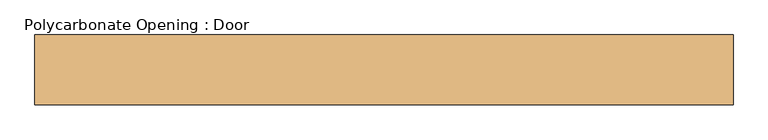
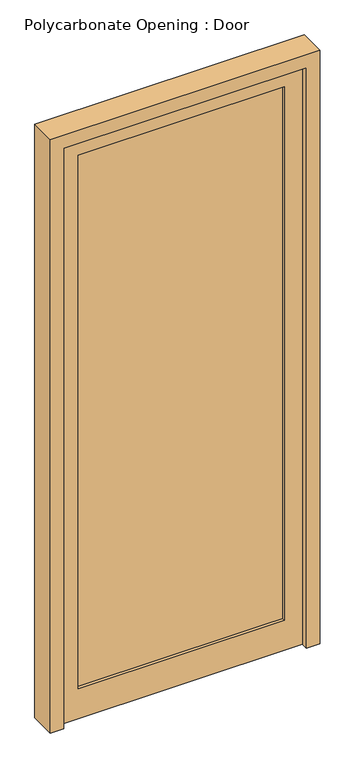
"""IFC4 building model written with IfcOpenShell, lengths in millimetres: door geometry, Polycarbonate Opening : Door."""

import ifcopenshell
import ifcopenshell.guid

model = None  # the IFC model being written
_history = None  # IfcOwnerHistory: only IFC2X3 demands one
_inside = {}  # id of a spatial element -> (the spatial element, [elements in it])
_under = {}  # id of a project, library or spatial element -> (it, [spatial elements below it])
_declared = {}  # id of a project -> (the project, [libraries it declares])
_typed = {}  # id of a type object -> (the type object, [elements of that type])
_made_of = {}  # id of a material, layer set ... -> (it, [elements and type objects made of it])


def new_model(schema):
    """Start an empty IFC model of exactly this schema.

    Asked for "IFC4X3", IfcOpenShell would pick the latest addendum, in which some entities
    have other attributes; the version numbers below select the first issue.
    IFC2X3 requires an IfcOwnerHistory on every rooted entity: one is made here for all.
    """
    global model, _history
    if schema == "IFC4X3":
        model = ifcopenshell.file(schema_version=(4, 3, 0, 0))
    else:
        model = ifcopenshell.file(schema=schema)
    _inside.clear()
    _under.clear()
    _declared.clear()
    _typed.clear()
    _made_of.clear()
    _history = None
    if model.schema == "IFC2X3":
        org = make("IfcOrganization", Name="unknown")
        user = make(
            "IfcPersonAndOrganization",
            ThePerson=make("IfcPerson", FamilyName="unknown"),
            TheOrganization=org,
        )
        app = make(
            "IfcApplication",
            ApplicationDeveloper=org,
            Version="unknown",
            ApplicationFullName="unknown",
            ApplicationIdentifier="unknown",
        )
        _history = make(
            "IfcOwnerHistory",
            OwningUser=user,
            OwningApplication=app,
            ChangeAction="ADDED",
            CreationDate=0,
        )
    return model


def make(cls, **values):
    """One entity of the class cls with the attributes given. An attribute that is None is left unset."""
    return model.create_entity(
        cls, **{name: value for name, value in values.items() if value is not None}
    )


def rooted(cls, **values):
    """An entity with a GlobalId (a new one), such as an element, a storey or a relation."""
    return make(cls, GlobalId=ifcopenshell.guid.new(), OwnerHistory=_history, **values)


def si_unit(unit_type, name, prefix=None):
    """IfcSIUnit, for example si_unit("LENGTHUNIT", "METRE", prefix="MILLI")."""
    return make("IfcSIUnit", UnitType=unit_type, Prefix=prefix, Name=name)


def assignment(units):
    """IfcUnitAssignment: the units of a project."""
    return None if units is None else make("IfcUnitAssignment", Units=units)


def point(xyz):
    """IfcCartesianPoint."""
    return None if xyz is None else make("IfcCartesianPoint", Coordinates=xyz)


def direction(xyz):
    """IfcDirection."""
    return None if xyz is None else make("IfcDirection", DirectionRatios=xyz)


def frame(location, z_axis=None, x_axis=None):
    """IfcAxis2Placement3D, a coordinate frame: its origin and axes. An axis left out is left unset."""
    return make(
        "IfcAxis2Placement3D",
        Location=point(location),
        Axis=direction(z_axis),
        RefDirection=direction(x_axis),
    )


def origin():
    """The frame at (0, 0, 0) with its axes left unset."""
    return frame((0.0, 0.0, 0.0))


def place(relative_to, where):
    """IfcLocalPlacement: puts the frame where relative to a parent placement (None: the world)."""
    return make(
        "IfcLocalPlacement", PlacementRelTo=relative_to, RelativePlacement=where
    )


def context(
    kind, dimensions, precision=None, world=None, true_north=None, identifier=None
):
    """IfcGeometricRepresentationContext, for example the 3D "Model" context."""
    return make(
        "IfcGeometricRepresentationContext",
        ContextIdentifier=identifier,
        ContextType=kind,
        CoordinateSpaceDimension=dimensions,
        Precision=precision,
        WorldCoordinateSystem=world,
        TrueNorth=true_north,
    )


def project(units=None, contexts=None):
    """IfcProject with its units and contexts."""
    return rooted(
        "IfcProject",
        Name="project",
        RepresentationContexts=contexts,
        UnitsInContext=assignment(units),
    )


def spatial(cls, under=None, at=None, **own):
    """A site, building, storey or space (cls), placed at a placement, below another one or the project."""
    s = rooted(cls, ObjectPlacement=at, **own)
    if under is not None:
        _under.setdefault(under.id(), (under, []))[1].append(s)
    return s


def polyline(points):
    """IfcPolyline through the points."""
    return make("IfcPolyline", Points=[point(p) for p in points])


def outline(outer, holes=None, kind="AREA"):
    """IfcArbitraryClosedProfileDef: a profile drawn as a closed curve; with holes, ...WithVoids."""
    if holes is None:
        return make("IfcArbitraryClosedProfileDef", ProfileType=kind, OuterCurve=outer)
    return make(
        "IfcArbitraryProfileDefWithVoids",
        ProfileType=kind,
        OuterCurve=outer,
        InnerCurves=holes,
    )


def extrude(swept, where, along, depth):
    """IfcExtrudedAreaSolid: the profile swept, set in the frame where, extruded along a direction by depth."""
    return make(
        "IfcExtrudedAreaSolid",
        SweptArea=swept,
        Position=where,
        ExtrudedDirection=direction(along),
        Depth=depth,
    )


def shape(context_of_items, identifier, shape_type, items):
    """IfcShapeRepresentation: the items that make up one representation, for example the "Body"."""
    return make(
        "IfcShapeRepresentation",
        ContextOfItems=context_of_items,
        RepresentationIdentifier=identifier,
        RepresentationType=shape_type,
        Items=items,
    )


def source(mapping_origin, context_of_items, identifier, shape_type, items):
    """IfcRepresentationMap: a shape defined once, which mapped items show again and again."""
    return make(
        "IfcRepresentationMap",
        MappingOrigin=mapping_origin,
        MappedRepresentation=shape(context_of_items, identifier, shape_type, items),
    )


def transform(
    local_origin,
    x_axis=None,
    y_axis=None,
    z_axis=None,
    scale=None,
    scale2=None,
    scale3=None,
    uniform=True,
):
    """IfcCartesianTransformationOperator3D, or its non-uniform kind. x_axis, y_axis, z_axis: its Axis1, 2, 3."""
    if uniform:
        return make(
            "IfcCartesianTransformationOperator3D",
            Axis1=direction(x_axis),
            Axis2=direction(y_axis),
            LocalOrigin=point(local_origin),
            Scale=scale,
            Axis3=direction(z_axis),
        )
    return make(
        "IfcCartesianTransformationOperator3DnonUniform",
        Axis1=direction(x_axis),
        Axis2=direction(y_axis),
        LocalOrigin=point(local_origin),
        Scale=scale,
        Axis3=direction(z_axis),
        Scale2=scale2,
        Scale3=scale3,
    )


def mapped(mapping_source, mapping_target):
    """IfcMappedItem: shows the shape of a source again, moved by a transform."""
    return make(
        "IfcMappedItem", MappingSource=mapping_source, MappingTarget=mapping_target
    )


def made_of(thing, what):
    """Note that an element or type object is made of a material, layer set ...; save() writes the relation."""
    if what is not None:
        _made_of.setdefault(what.id(), (what, []))[1].append(thing)
    return thing


def element(
    cls,
    number,
    at=None,
    inside=None,
    cuts=None,
    type_object=None,
    material=None,
    context=None,
    identifier="Body",
    shape_type=None,
    held_by="IfcProductDefinitionShape",
    body=None,
    shapes=None,
    **own,
):
    """One element of the class cls, such as IfcWall. Its Tag is "e" and its number.

    at: its placement. inside: the storey or other place that contains it. cuts: it is an
    opening in that element (IfcRelVoidsElement). A single representation is given by context,
    identifier, shape_type and body (its items); several are given by shapes. held_by: the class
    of the entity that holds the representations. save() writes the other relations.
    """
    e = rooted(cls, Tag="e%d" % number, ObjectPlacement=at, **own)
    if body is not None:
        shapes = [shape(context, identifier, shape_type, body)]
    if shapes is not None:
        e.Representation = make(held_by, Representations=shapes)
    if inside is not None:
        _inside.setdefault(inside.id(), (inside, []))[1].append(e)
    if cuts is not None:
        rooted(
            "IfcRelVoidsElement", RelatingBuildingElement=cuts, RelatedOpeningElement=e
        )
    if type_object is not None:
        _typed.setdefault(type_object.id(), (type_object, []))[1].append(e)
    return made_of(e, material)


def aggregate(whole, parts):
    """IfcRelAggregates: a whole, such as a stair, and the parts it consists of."""
    return rooted("IfcRelAggregates", RelatingObject=whole, RelatedObjects=parts)


def save(model, path):
    """Write the relations noted so far, then the file.

    IfcRelAggregates (storeys below a building ...), IfcRelContainedInSpatialStructure (elements
    in a storey), IfcRelDefinesByType, IfcRelAssociatesMaterial and IfcRelDeclares: one each for
    every whole, place, type object, material and project.
    """
    for whole, parts in _under.values():
        aggregate(whole, parts)
    for where, things in _inside.values():
        rooted(
            "IfcRelContainedInSpatialStructure",
            RelatedElements=things,
            RelatingStructure=where,
        )
    for kind, things in _typed.values():
        rooted("IfcRelDefinesByType", RelatedObjects=things, RelatingType=kind)
    for what, things in _made_of.values():
        rooted("IfcRelAssociatesMaterial", RelatedObjects=things, RelatingMaterial=what)
    for by, libraries in _declared.values():
        rooted("IfcRelDeclares", RelatingContext=by, RelatedDefinitions=libraries)
    model.write(path)


def polycarbonate_opening_door_04931fee(model_context):
    return source(origin(), model_context, "Body", "SweptSolid", [
        extrude(outline(polyline([(457.2, 0.0), (-457.2, 0.0), (-457.2, 25.4), (457.2, 25.4), (457.2, 0.0)])), frame((0.0, 0.0, 50.8), z_axis=(0.0, 0.0, 1.0), x_axis=(1.0, 0.0, 0.0)), (0.0, 0.0, 1.0), 2260.6),
        extrude(outline(polyline([(2311.4, -457.2), (0.0, -457.2), (0.0, 457.2), (2311.4, 457.2), (2311.4, -457.2)]), holes=[polyline([(119.0625, 388.9375), (119.0625, -388.9375), (2243.1375, -388.9375), (2243.1375, 388.9375), (119.0625, 388.9375)])]), frame((0.0, -12.7, 0.0), z_axis=(0.0, 1.0, 0.0), x_axis=(0.0, 0.0, 1.0)), (0.0, 0.0, 1.0), 50.8),
        extrude(outline(polyline([(2362.2, 508.0), (2362.2, -508.0), (0.0, -508.0), (0.0, -457.2), (2311.4, -457.2), (2311.4, 457.2), (0.0, 457.2), (0.0, 508.0), (2362.2, 508.0)])), frame((0.0, -38.1, 0.0), z_axis=(0.0, 1.0, 0.0), x_axis=(0.0, 0.0, 1.0)), (0.0, 0.0, 1.0), 101.6),
    ])


if __name__ == "__main__":
    model = new_model("IFC4")
    model_context = context("Model", 3, world=origin())
    ifc_project = project(units=[si_unit("LENGTHUNIT", "METRE", prefix="MILLI")], contexts=[model_context])
    site = spatial("IfcSite", under=ifc_project)
    building = spatial("IfcBuilding", under=site)
    placement = place(None, origin())
    polycarbonate_opening_door_shape = polycarbonate_opening_door_04931fee(model_context)
    element("IfcDoor", 1, ObjectType="Polycarbonate Opening : Door", at=placement, inside=building, context=model_context, shape_type="MappedRepresentation", body=[
        mapped(polycarbonate_opening_door_shape, transform((0.0, 0.0, 0.0), x_axis=(1.0, 0.0, 0.0), y_axis=(0.0, 1.0, 0.0), z_axis=(0.0, 0.0, 1.0))),
    ])
    save(model, "model.ifc")

# Revit data of these elements
# Type "Polycarbonate Opening : Door"
#   Type Mark = "60"
#   OD_DS_Door_Material = "ALUM./GLAZING"
#   OD_DS_Door_Type = "STOREFRONT (NARROW STILE)"
#   OD_DS_Lockset = "ENTRY LOCK (INSIDE ADA LEVER ALWAYS ACTIVE)"
#   Analytic Construction = "<None>"
#   offset [instance default] = 0' - 0 1/2"
#   Stile = 0' - 2 11/16"
#   Mullion Width = 0' - 2"
#   Mullion Depth = 0' - 4"
#   Opening Size [instance default] = 5' - 1.50212"
#   Door Width [instance default] = 5' - 1.50212"
#   Window ON/OFF = yes
#   Door On/Off = no
#   Mullion Material = KAWNEER 260 INSULCLADTM THERMAL ENTRANCE - CLEAR ANODIZED ALUM.
#   Glass Material = TEMPERED INSULATED GLAZING (CARDINAL GLASS LoĒ²-240\nOR EQUIVALENT)
#   Door Material = KAWNEER 260 INSULCLADTM THERMAL ENTRANCE - CLEAR ANODIZED ALUM.
# Element 1 (IfcDoor, "Polycarbonate Opening : Door")
#   Materials on its faces: "KAWNEER 260 INSULCLADTM THERMAL ENTRANCE - CLEAR ANODIZED ALUM.", "TEMPERED INSULATED GLAZING (CARDINAL GLASS LoĒ²-240\nOR EQUIVALENT)"
# Materials
#   "KAWNEER 260 INSULCLADTM THERMAL ENTRANCE - CLEAR ANODIZED ALUM.": class "Metal", colour RGB 244 244 244, transparency 0, Description = "Aluminum 6061", Cost = 0
#   "TEMPERED INSULATED GLAZING (CARDINAL GLASS LoĒ²-240\nOR EQUIVALENT)": class "Glass", colour RGB 196 205 210, transparency 0.85, Description = "Soda Lime Glass", Cost = 0
